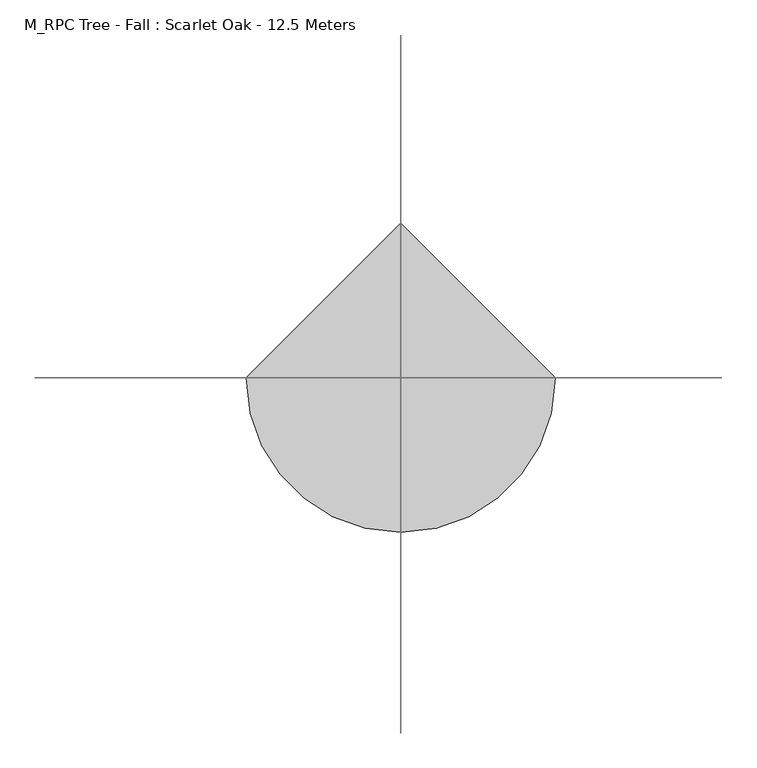
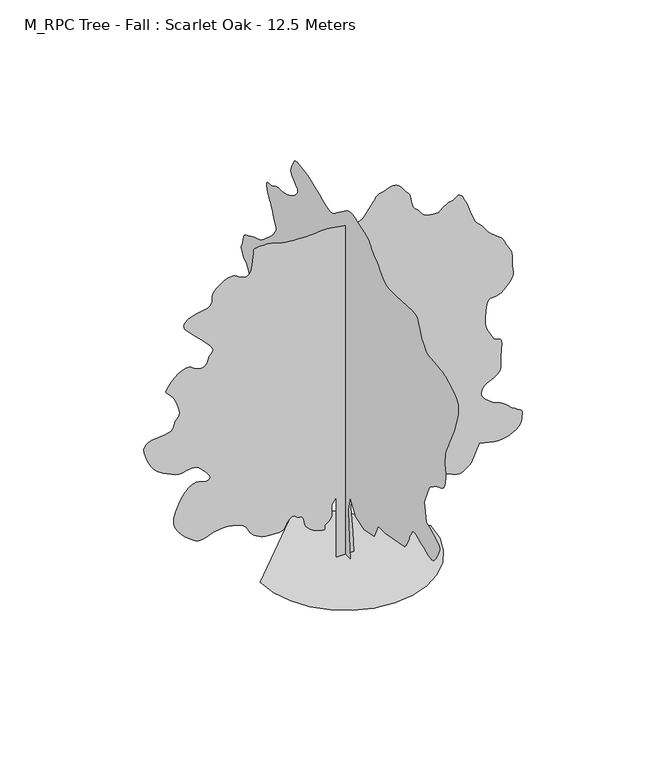
# IFC4 building model written with IfcOpenShell, lengths in millimetres: geographic element geometry, M_RPC Tree - Fall : Scarlet Oak - 12.5 Meters.
# Revit data of these elements (continued)
# Type "M_RPC Tree - Fall : Scarlet Oak - 12.5 Meters"
#   built-in parameter 1005198 = "{2, 15},{39, RPC-16-FXGN-QL00-PPP3-E000-ST1L-LVER-AU},{1, 0},{1, 0},{2, 13},{1, 8},{5, Color},{1, 0},{1, 0},{3, 0.8},{3, 0.8},{3, 0.8},{1, 8},{7, BBoxMin},{1, 0},{1, 0},{1, 0},{1, 0},{1, 0},{1, 8},{7, BBoxMax},{1, 0},{1, 0},{1, 0},{1, 0},{1, 0},{2, 11},{9, RPCTypeId},{1, 0},{1, 0},{39, RPC-16-FXGN-QL00-PPP3-E000-ST1L-LVER-AU},{1, 6},{14, RPCPlantHeight},{1, 0},{1, 0},{7, 41.0105},{2, 11},{7, keyword},{1, 0},{1, 0},{39, :RPCs:Fall Trees [General]:Geometry:RPC},{2, 11},{8, category},{1, 0},{1, 0},{20, Fall Trees [General]},{2, 11},{12, LocalizedUID},{1, 0},{1, 0},{18, Scarlet Oak [Fall]},{2, 14},{6, Height},{1, 0},{1, 0},{7, 41.0105},{1, 2},{16, Cast Reflections},{1, 0},{1, 0},{1, 0},{1, 2},{12, Cast Shadows},{1, 0},{1, 0},{1, 1},{1, 2},{9, Lock View},{1, 0},{1, 0},{1, 0},{1, 4},{5, ViewC},{1, 0},{1, 0},{1, 0},{21, assetlibrary_base.fbx},{1, 5},"
#   built-in parameter 1005195 = "RPC-16-FXGN-QL00-PPP3-E000-ST1L-LVER-AU"
#   Type Comments = "Scarlet Oak"
#   Height = 12.5 m
#   Default Elevation = 0
